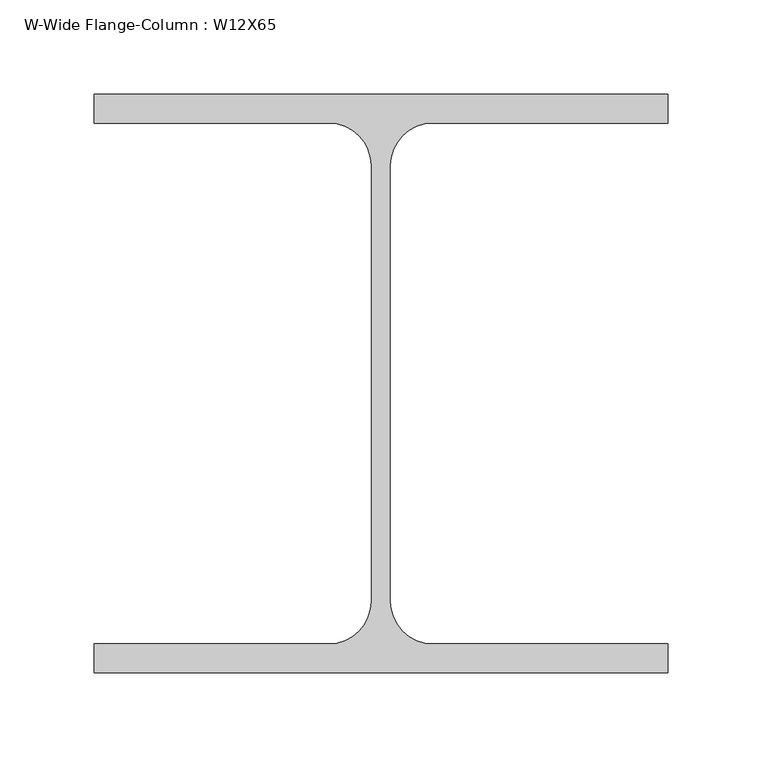
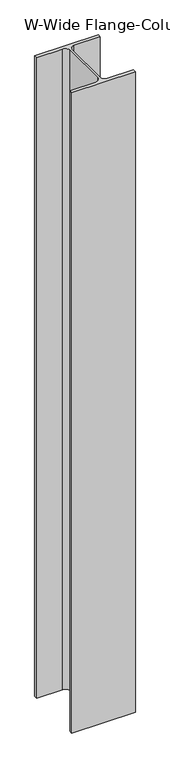
"""IFC4 building model written with IfcOpenShell, lengths in millimetres: column geometry, W-Wide Flange-Column : W12X65."""

from ifc_helpers import new_model, si_unit, point, frame, frame_2d, origin, place, context, project, spatial, polyline, circle_curve, trimmed, segment, composite_curve, outline, extrude, source, transform, mapped, element, save


def w_wide_flange_column_w12x65_1fdfdda2(model_context):
    return source(origin(), model_context, "Body", "SweptSolid", [
        extrude(outline(composite_curve([segment(polyline([(152.4, 153.67), (152.4, 138.303), (27.686, 138.303)]), True, "CONTINUOUS"), segment(trimmed(circle_curve(frame_2d((27.686, 115.57)), 22.733), [point((27.686, 138.303))], [point((4.953, 115.57))], True, "CARTESIAN"), True, "CONTINUOUS"), segment(polyline([(4.953, 115.57), (4.953, -115.57)]), True, "CONTINUOUS"), segment(trimmed(circle_curve(frame_2d((27.686, -115.57)), 22.733), [point((4.953, -115.57))], [point((27.686, -138.303))], True, "CARTESIAN"), True, "CONTINUOUS"), segment(polyline([(27.686, -138.303), (152.4, -138.303), (152.4, -153.67), (-152.4, -153.67), (-152.4, -138.303), (-27.686, -138.303)]), True, "CONTINUOUS"), segment(trimmed(circle_curve(frame_2d((-27.686, -115.57)), 22.733), [point((-27.686, -138.303))], [point((-4.953, -115.57))], True, "CARTESIAN"), True, "CONTINUOUS"), segment(polyline([(-4.953, -115.57), (-4.953, 115.57)]), True, "CONTINUOUS"), segment(trimmed(circle_curve(frame_2d((-27.686, 115.57)), 22.733), [point((-4.953, 115.57))], [point((-27.686, 138.303))], True, "CARTESIAN"), True, "CONTINUOUS"), segment(polyline([(-27.686, 138.303), (-152.4, 138.303), (-152.4, 153.67), (152.4, 153.67)]), True, "CONTINUOUS")], self_intersect=False)), frame((0.0, 0.0, 9163.05), z_axis=(0.0, 0.0, 1.0), x_axis=(1.0, 0.0, 0.0)), (0.0, 0.0, 1.0), 3244.85),
    ])


if __name__ == "__main__":
    model = new_model("IFC4")
    model_context = context("Model", 3, world=origin())
    ifc_project = project(units=[si_unit("LENGTHUNIT", "METRE", prefix="MILLI")], contexts=[model_context])
    site = spatial("IfcSite", under=ifc_project)
    building = spatial("IfcBuilding", under=site)
    placement = place(None, origin())
    w_wide_flange_column_w12x65_shape = w_wide_flange_column_w12x65_1fdfdda2(model_context)
    element("IfcColumn", 1, ObjectType="W-Wide Flange-Column : W12X65", at=placement, inside=building, context=model_context, shape_type="MappedRepresentation", body=[
        mapped(w_wide_flange_column_w12x65_shape, transform((0.0, 0.0, 0.0), x_axis=(1.0, 0.0, 0.0), y_axis=(0.0, 1.0, 0.0), z_axis=(0.0, 0.0, 1.0))),
    ])
    save(model, "model.ifc")

# Revit data of these elements
# Type "W-Wide Flange-Column : W12X65"
#   Assembly Code = "B10"
#   W = 65
#   bf = 1' - 0"
#   d = 1' - 0.1"
#   k = 0' - 1 1/2"
#   kr = 0' - 0.895"
#   tf = 0' - 0.605"
#   tw = 0' - 0.39"
#   A = 0.132639 SF
#   Structural Material [instance default] = Steel ASTM A992
# Element 1 (IfcColumn, "W-Wide Flange-Column : W12X65")
#   Materials on its faces: "Steel ASTM A992"
# Materials
#   "Steel ASTM A992": class "Metal", colour RGB 199 199 199, transparency 0, Description = "Structural steel 50ksi", Cost = 0
